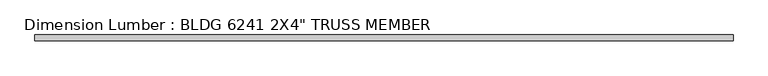
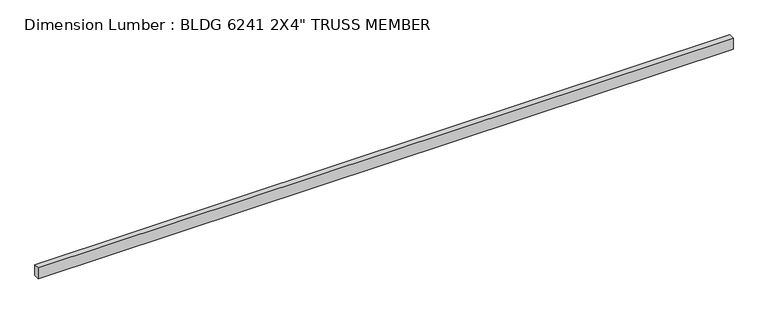
"""IFC4 building model written with IfcOpenShell, lengths in millimetres: beam geometry."""

from ifc_helpers import new_model, si_unit, frame, origin, place, context, project, spatial, polyline, outline, extrude, source, transform, mapped, element, save


def beam_5c93efd5(model_context):
    return source(origin(), model_context, "Body", "SweptSolid", [
        extrude(outline(polyline([(3063.8749994, 25.4), (3063.8749994, -25.4), (-3063.8749994, -25.4), (-3063.8749994, 25.4), (3063.8749994, 25.4)])), frame((0.0, 0.0, -50.8), z_axis=(0.0, 0.0, 1.0), x_axis=(1.0, 0.0, 0.0)), (0.0, 0.0, 1.0), 101.6),
    ])


if __name__ == "__main__":
    model = new_model("IFC4")
    model_context = context("Model", 3, world=origin())
    ifc_project = project(units=[si_unit("LENGTHUNIT", "METRE", prefix="MILLI")], contexts=[model_context])
    site = spatial("IfcSite", under=ifc_project)
    building = spatial("IfcBuilding", under=site)
    placement = place(None, origin())
    beam_shape = beam_5c93efd5(model_context)
    element("IfcBeam", 1, ObjectType="Dimension Lumber : BLDG 6241 2X4\" TRUSS MEMBER", at=placement, inside=building, context=model_context, shape_type="MappedRepresentation", body=[
        mapped(beam_shape, transform((0.0, 0.0, 0.0), x_axis=(1.0, 0.0, 0.0), y_axis=(0.0, 1.0, 0.0), z_axis=(0.0, 0.0, 1.0))),
    ])
    save(model, "model.ifc")

# Revit data of these elements
# Type "Dimension Lumber : BLDG 6241 2X4\" TRUSS MEMBER"
#   Assembly Code = "B10"
#   A = 0.273472 SF
#   Length [instance default] = 5' - 0"
#   b = 0' - 2"
#   d = 0' - 4"
#   Structural Material [instance default] = Softwood, Lumber
# Element 1 (IfcBeam, "Dimension Lumber : BLDG 6241 2X4\" TRUSS MEMBER")
#   Materials on its faces: "Softwood, Lumber"
# Materials
#   "Softwood, Lumber": class "Wood", colour RGB 223 192 134, transparency 0, Description = "Pinus Echinata", Cost = 0
